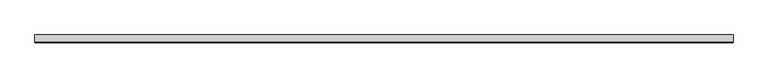
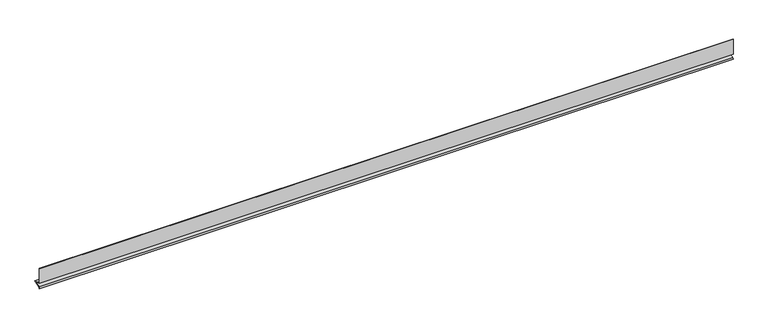
"""IFC4 building model written with IfcOpenShell, lengths in millimetres: proxy geometry, Metal profile005 1238 : Metal profile005 1238."""

from ifc_helpers import new_model, si_unit, frame, origin, place, context, project, spatial, polyline, outline, extrude, source, transform, mapped, element, save


def generic_models_58486194(model_context):
    return source(origin(), model_context, "Body", "SweptSolid", [
        extrude(outline(polyline([(9752.5625834, 36529.4059354), (9753.5257785, 36534.5206858), (9770.6373811, 36540.0208437), (9752.5625834, 36545.8306002), (9752.5625834, 36590.8208437), (9753.8325834, 36590.8208437), (9753.8325834, 36546.7563795), (9774.7875834, 36540.0208437), (9754.6339669, 36533.5428956), (9753.8106459, 36529.1709038), (9752.5625834, 36529.4059354)])), frame((3694.2883192, 0.0, 0.0), z_axis=(1.0, 0.0, 0.0), x_axis=(0.0, 1.0, 0.0)), (0.0, 0.0, 1.0), 2000.0),
    ])


if __name__ == "__main__":
    model = new_model("IFC4")
    model_context = context("Model", 3, world=origin())
    ifc_project = project(units=[si_unit("LENGTHUNIT", "METRE", prefix="MILLI")], contexts=[model_context])
    site = spatial("IfcSite", under=ifc_project)
    building = spatial("IfcBuilding", under=site)
    placement = place(None, origin())
    generic_models_shape = generic_models_58486194(model_context)
    element("IfcBuildingElementProxy", 1, Name="Metal profile005 1238 : Metal profile005 1238", ObjectType="Metal profile005 1238 : Metal profile005 1238", at=placement, inside=building, context=model_context, shape_type="MappedRepresentation", body=[
        mapped(generic_models_shape, transform((0.0, 0.0, 0.0), x_axis=(1.0, 0.0, 0.0), y_axis=(0.0, 1.0, 0.0), z_axis=(0.0, 0.0, 1.0))),
    ])
    save(model, "model.ifc")

# Revit data of these elements
# Type "Metal profile005 1238 : Metal profile005 1238"
#   NameOverride = "Metal profile005"
# Element 1 (IfcBuildingElementProxy, "Metal profile005 1238 : Metal profile005 1238")
#   Materials on its faces: "16 GA. COPPER WEEP SCREED W/ MIN 3 1/2\" ATTACHMENT FLANGE - LAP UNDERLAYMENT OVER WEED SCREED"
# Materials
#   "16 GA. COPPER WEEP SCREED W/ MIN 3 1/2\" ATTACHMENT FLANGE - LAP UNDERLAYMENT OVER WEED SCREED": class "Unassigned", colour RGB 255 237 20, transparency 0
